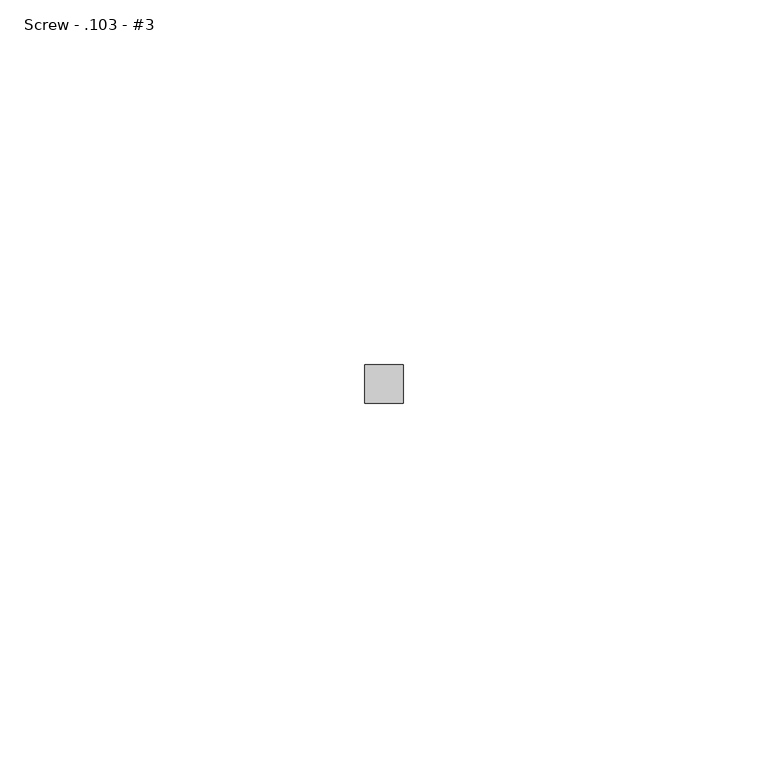
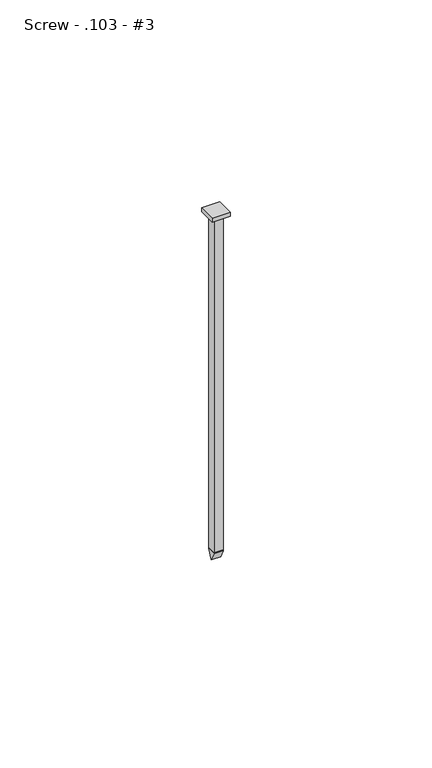
"""IFC4 building model written with IfcOpenShell, lengths in millimetres: fastener geometry, 060523 - W_P_C - Fastenings - Generic - SQUARE : Screw - .103 - #3."""

import ifcopenshell
import ifcopenshell.guid

model = None  # the IFC model being written
_history = None  # IfcOwnerHistory: only IFC2X3 demands one
_inside = {}  # id of a spatial element -> (the spatial element, [elements in it])
_under = {}  # id of a project, library or spatial element -> (it, [spatial elements below it])
_declared = {}  # id of a project -> (the project, [libraries it declares])
_typed = {}  # id of a type object -> (the type object, [elements of that type])
_made_of = {}  # id of a material, layer set ... -> (it, [elements and type objects made of it])


def new_model(schema):
    """Start an empty IFC model of exactly this schema.

    Asked for "IFC4X3", IfcOpenShell would pick the latest addendum, in which some entities
    have other attributes; the version numbers below select the first issue.
    IFC2X3 requires an IfcOwnerHistory on every rooted entity: one is made here for all.
    """
    global model, _history
    if schema == "IFC4X3":
        model = ifcopenshell.file(schema_version=(4, 3, 0, 0))
    else:
        model = ifcopenshell.file(schema=schema)
    _inside.clear()
    _under.clear()
    _declared.clear()
    _typed.clear()
    _made_of.clear()
    _history = None
    if model.schema == "IFC2X3":
        org = make("IfcOrganization", Name="unknown")
        user = make(
            "IfcPersonAndOrganization",
            ThePerson=make("IfcPerson", FamilyName="unknown"),
            TheOrganization=org,
        )
        app = make(
            "IfcApplication",
            ApplicationDeveloper=org,
            Version="unknown",
            ApplicationFullName="unknown",
            ApplicationIdentifier="unknown",
        )
        _history = make(
            "IfcOwnerHistory",
            OwningUser=user,
            OwningApplication=app,
            ChangeAction="ADDED",
            CreationDate=0,
        )
    return model


def make(cls, **values):
    """One entity of the class cls with the attributes given. An attribute that is None is left unset."""
    return model.create_entity(
        cls, **{name: value for name, value in values.items() if value is not None}
    )


def rooted(cls, **values):
    """An entity with a GlobalId (a new one), such as an element, a storey or a relation."""
    return make(cls, GlobalId=ifcopenshell.guid.new(), OwnerHistory=_history, **values)


def si_unit(unit_type, name, prefix=None):
    """IfcSIUnit, for example si_unit("LENGTHUNIT", "METRE", prefix="MILLI")."""
    return make("IfcSIUnit", UnitType=unit_type, Prefix=prefix, Name=name)


def assignment(units):
    """IfcUnitAssignment: the units of a project."""
    return None if units is None else make("IfcUnitAssignment", Units=units)


def point(xyz):
    """IfcCartesianPoint."""
    return None if xyz is None else make("IfcCartesianPoint", Coordinates=xyz)


def direction(xyz):
    """IfcDirection."""
    return None if xyz is None else make("IfcDirection", DirectionRatios=xyz)


def frame(location, z_axis=None, x_axis=None):
    """IfcAxis2Placement3D, a coordinate frame: its origin and axes. An axis left out is left unset."""
    return make(
        "IfcAxis2Placement3D",
        Location=point(location),
        Axis=direction(z_axis),
        RefDirection=direction(x_axis),
    )


def origin():
    """The frame at (0, 0, 0) with its axes left unset."""
    return frame((0.0, 0.0, 0.0))


def origin_with_axes():
    """The frame at (0, 0, 0) with the z axis (0, 0, 1) and the x axis (1, 0, 0) written out."""
    return frame((0.0, 0.0, 0.0), z_axis=(0.0, 0.0, 1.0), x_axis=(1.0, 0.0, 0.0))


def place(relative_to, where):
    """IfcLocalPlacement: puts the frame where relative to a parent placement (None: the world)."""
    return make(
        "IfcLocalPlacement", PlacementRelTo=relative_to, RelativePlacement=where
    )


def context(
    kind, dimensions, precision=None, world=None, true_north=None, identifier=None
):
    """IfcGeometricRepresentationContext, for example the 3D "Model" context."""
    return make(
        "IfcGeometricRepresentationContext",
        ContextIdentifier=identifier,
        ContextType=kind,
        CoordinateSpaceDimension=dimensions,
        Precision=precision,
        WorldCoordinateSystem=world,
        TrueNorth=true_north,
    )


def project(units=None, contexts=None):
    """IfcProject with its units and contexts."""
    return rooted(
        "IfcProject",
        Name="project",
        RepresentationContexts=contexts,
        UnitsInContext=assignment(units),
    )


def spatial(cls, under=None, at=None, **own):
    """A site, building, storey or space (cls), placed at a placement, below another one or the project."""
    s = rooted(cls, ObjectPlacement=at, **own)
    if under is not None:
        _under.setdefault(under.id(), (under, []))[1].append(s)
    return s


def polyline(points):
    """IfcPolyline through the points."""
    return make("IfcPolyline", Points=[point(p) for p in points])


def outline(outer, holes=None, kind="AREA"):
    """IfcArbitraryClosedProfileDef: a profile drawn as a closed curve; with holes, ...WithVoids."""
    if holes is None:
        return make("IfcArbitraryClosedProfileDef", ProfileType=kind, OuterCurve=outer)
    return make(
        "IfcArbitraryProfileDefWithVoids",
        ProfileType=kind,
        OuterCurve=outer,
        InnerCurves=holes,
    )


def extrude(swept, where, along, depth):
    """IfcExtrudedAreaSolid: the profile swept, set in the frame where, extruded along a direction by depth."""
    return make(
        "IfcExtrudedAreaSolid",
        SweptArea=swept,
        Position=where,
        ExtrudedDirection=direction(along),
        Depth=depth,
    )


def shape(context_of_items, identifier, shape_type, items):
    """IfcShapeRepresentation: the items that make up one representation, for example the "Body"."""
    return make(
        "IfcShapeRepresentation",
        ContextOfItems=context_of_items,
        RepresentationIdentifier=identifier,
        RepresentationType=shape_type,
        Items=items,
    )


def source(mapping_origin, context_of_items, identifier, shape_type, items):
    """IfcRepresentationMap: a shape defined once, which mapped items show again and again."""
    return make(
        "IfcRepresentationMap",
        MappingOrigin=mapping_origin,
        MappedRepresentation=shape(context_of_items, identifier, shape_type, items),
    )


def transform(
    local_origin,
    x_axis=None,
    y_axis=None,
    z_axis=None,
    scale=None,
    scale2=None,
    scale3=None,
    uniform=True,
):
    """IfcCartesianTransformationOperator3D, or its non-uniform kind. x_axis, y_axis, z_axis: its Axis1, 2, 3."""
    if uniform:
        return make(
            "IfcCartesianTransformationOperator3D",
            Axis1=direction(x_axis),
            Axis2=direction(y_axis),
            LocalOrigin=point(local_origin),
            Scale=scale,
            Axis3=direction(z_axis),
        )
    return make(
        "IfcCartesianTransformationOperator3DnonUniform",
        Axis1=direction(x_axis),
        Axis2=direction(y_axis),
        LocalOrigin=point(local_origin),
        Scale=scale,
        Axis3=direction(z_axis),
        Scale2=scale2,
        Scale3=scale3,
    )


def mapped(mapping_source, mapping_target):
    """IfcMappedItem: shows the shape of a source again, moved by a transform."""
    return make(
        "IfcMappedItem", MappingSource=mapping_source, MappingTarget=mapping_target
    )


def made_of(thing, what):
    """Note that an element or type object is made of a material, layer set ...; save() writes the relation."""
    if what is not None:
        _made_of.setdefault(what.id(), (what, []))[1].append(thing)
    return thing


def element(
    cls,
    number,
    at=None,
    inside=None,
    cuts=None,
    type_object=None,
    material=None,
    context=None,
    identifier="Body",
    shape_type=None,
    held_by="IfcProductDefinitionShape",
    body=None,
    shapes=None,
    **own,
):
    """One element of the class cls, such as IfcWall. Its Tag is "e" and its number.

    at: its placement. inside: the storey or other place that contains it. cuts: it is an
    opening in that element (IfcRelVoidsElement). A single representation is given by context,
    identifier, shape_type and body (its items); several are given by shapes. held_by: the class
    of the entity that holds the representations. save() writes the other relations.
    """
    e = rooted(cls, Tag="e%d" % number, ObjectPlacement=at, **own)
    if body is not None:
        shapes = [shape(context, identifier, shape_type, body)]
    if shapes is not None:
        e.Representation = make(held_by, Representations=shapes)
    if inside is not None:
        _inside.setdefault(inside.id(), (inside, []))[1].append(e)
    if cuts is not None:
        rooted(
            "IfcRelVoidsElement", RelatingBuildingElement=cuts, RelatedOpeningElement=e
        )
    if type_object is not None:
        _typed.setdefault(type_object.id(), (type_object, []))[1].append(e)
    return made_of(e, material)


def aggregate(whole, parts):
    """IfcRelAggregates: a whole, such as a stair, and the parts it consists of."""
    return rooted("IfcRelAggregates", RelatingObject=whole, RelatedObjects=parts)


def save(model, path):
    """Write the relations noted so far, then the file.

    IfcRelAggregates (storeys below a building ...), IfcRelContainedInSpatialStructure (elements
    in a storey), IfcRelDefinesByType, IfcRelAssociatesMaterial and IfcRelDeclares: one each for
    every whole, place, type object, material and project.
    """
    for whole, parts in _under.values():
        aggregate(whole, parts)
    for where, things in _inside.values():
        rooted(
            "IfcRelContainedInSpatialStructure",
            RelatedElements=things,
            RelatingStructure=where,
        )
    for kind, things in _typed.values():
        rooted("IfcRelDefinesByType", RelatedObjects=things, RelatingType=kind)
    for what, things in _made_of.values():
        rooted("IfcRelAssociatesMaterial", RelatedObjects=things, RelatingMaterial=what)
    for by, libraries in _declared.values():
        rooted("IfcRelDeclares", RelatingContext=by, RelatedDefinitions=libraries)
    model.write(path)


def screw_103_3_3ef0f881(model_context):
    return source(origin(), model_context, "Body", "SweptSolid", [
        extrude(outline(polyline([(0.0, -104.2162), (-1.3081, -101.6), (1.3081, -101.6), (0.0, -104.2162)])), frame((-1.3081, 0.0, 0.0), z_axis=(1.0, 0.0, 0.0), x_axis=(0.0, 1.0, 0.0)), (0.0, 0.0, 1.0), 2.6162),
        extrude(outline(polyline([(-2.6162, -2.6162), (-2.6162, 2.6162), (2.6162, 2.6162), (2.6162, -2.6162), (-2.6162, -2.6162)])), origin_with_axes(), (0.0, 0.0, 1.0), 1.3081),
        extrude(outline(polyline([(-1.3081, 1.3081), (1.3081, 1.3081), (1.3081, -1.3081), (-1.3081, -1.3081), (-1.3081, 1.3081)])), frame((0.0, 0.0, -101.6), z_axis=(0.0, 0.0, 1.0), x_axis=(1.0, 0.0, 0.0)), (0.0, 0.0, 1.0), 101.6),
    ])


if __name__ == "__main__":
    model = new_model("IFC4")
    model_context = context("Model", 3, world=origin())
    ifc_project = project(units=[si_unit("LENGTHUNIT", "METRE", prefix="MILLI")], contexts=[model_context])
    site = spatial("IfcSite", under=ifc_project)
    building = spatial("IfcBuilding", under=site)
    placement = place(None, origin())
    screw_103_3_shape = screw_103_3_3ef0f881(model_context)
    element("IfcFastener", 1, ObjectType="060523 - W_P_C - Fastenings - Generic - SQUARE : Screw - .103 - #3", at=placement, inside=building, context=model_context, shape_type="MappedRepresentation", body=[
        mapped(screw_103_3_shape, transform((0.0, 0.0, 0.0), x_axis=(1.0, 0.0, 0.0), y_axis=(0.0, 1.0, 0.0), z_axis=(0.0, 0.0, 1.0))),
    ])
    save(model, "model.ifc")

# Revit data of these elements
# Type "060523 - W_P_C - Fastenings - Generic - SQUARE : Screw - .103 - #3"
#   Washer_Thickness = 0' - 0.00333"
#   Washer Radius = 0' - 0.0615"
#   Washer Offset - Head = 0' - 0"
#   Washer Offset = 0' - 0"
#   Thickness_of_Substrate [instance default] = 0' - 1"
#   Side = 0' - 0 37/64"
#   Radius = 0' - 0.0515"
#   Length [instance default] = 0' - 4"
#   Head Size = 0' - 1"
#   Head Radius = 0' - 0 1/2"
#   Head Height = 0' - 0.01"
#   Double Diameter = 0' - 0.206"
#   Diameter = 0' - 0.103"
#   Default Elevation = 4' - 0"
#   Washer_Nut_Visibility = no
#   Washer_Head_Visibility = no
#   Round_Head_Visibility = yes
#   Point Visibility = yes
#   Nut_Visibility = no
#   Hex_Head_Visiblilty = no
#   Washer Material = none
#   Bolt Material (Size) = AT SILL - FASTENER AT 24" O.C.
# Materials
#   "AT SILL - FASTENER AT 24\" O.C.": class "Generic", colour RGB 120 120 120, transparency 0, Cost = 0
